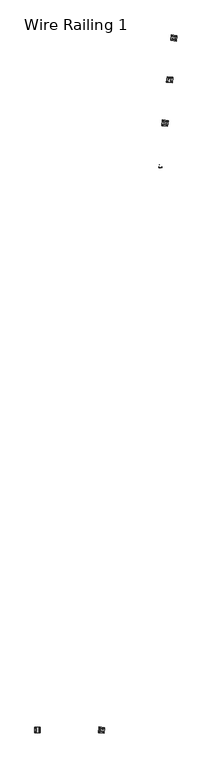
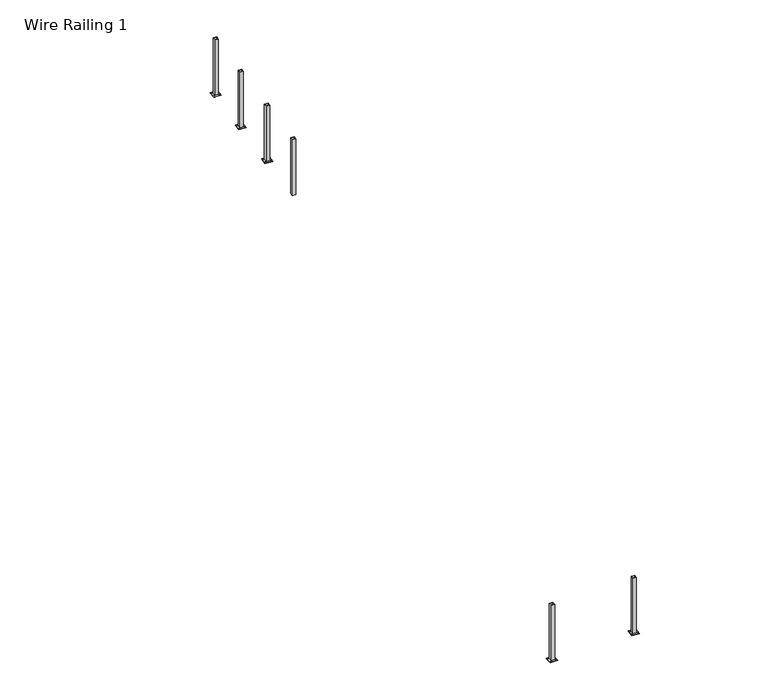
"""IFC4 building model written with IfcOpenShell, lengths in millimetres: railing geometry, Wire Railing 1."""

import ifcopenshell
import ifcopenshell.guid

model = None  # the IFC model being written
_history = None  # IfcOwnerHistory: only IFC2X3 demands one
_inside = {}  # id of a spatial element -> (the spatial element, [elements in it])
_under = {}  # id of a project, library or spatial element -> (it, [spatial elements below it])
_declared = {}  # id of a project -> (the project, [libraries it declares])
_typed = {}  # id of a type object -> (the type object, [elements of that type])
_made_of = {}  # id of a material, layer set ... -> (it, [elements and type objects made of it])


def new_model(schema):
    """Start an empty IFC model of exactly this schema.

    Asked for "IFC4X3", IfcOpenShell would pick the latest addendum, in which some entities
    have other attributes; the version numbers below select the first issue.
    IFC2X3 requires an IfcOwnerHistory on every rooted entity: one is made here for all.
    """
    global model, _history
    if schema == "IFC4X3":
        model = ifcopenshell.file(schema_version=(4, 3, 0, 0))
    else:
        model = ifcopenshell.file(schema=schema)
    _inside.clear()
    _under.clear()
    _declared.clear()
    _typed.clear()
    _made_of.clear()
    _history = None
    if model.schema == "IFC2X3":
        org = make("IfcOrganization", Name="unknown")
        user = make(
            "IfcPersonAndOrganization",
            ThePerson=make("IfcPerson", FamilyName="unknown"),
            TheOrganization=org,
        )
        app = make(
            "IfcApplication",
            ApplicationDeveloper=org,
            Version="unknown",
            ApplicationFullName="unknown",
            ApplicationIdentifier="unknown",
        )
        _history = make(
            "IfcOwnerHistory",
            OwningUser=user,
            OwningApplication=app,
            ChangeAction="ADDED",
            CreationDate=0,
        )
    return model


def make(cls, **values):
    """One entity of the class cls with the attributes given. An attribute that is None is left unset."""
    return model.create_entity(
        cls, **{name: value for name, value in values.items() if value is not None}
    )


def rooted(cls, **values):
    """An entity with a GlobalId (a new one), such as an element, a storey or a relation."""
    return make(cls, GlobalId=ifcopenshell.guid.new(), OwnerHistory=_history, **values)


def si_unit(unit_type, name, prefix=None):
    """IfcSIUnit, for example si_unit("LENGTHUNIT", "METRE", prefix="MILLI")."""
    return make("IfcSIUnit", UnitType=unit_type, Prefix=prefix, Name=name)


def assignment(units):
    """IfcUnitAssignment: the units of a project."""
    return None if units is None else make("IfcUnitAssignment", Units=units)


def point(xyz):
    """IfcCartesianPoint."""
    return None if xyz is None else make("IfcCartesianPoint", Coordinates=xyz)


def direction(xyz):
    """IfcDirection."""
    return None if xyz is None else make("IfcDirection", DirectionRatios=xyz)


def frame(location, z_axis=None, x_axis=None):
    """IfcAxis2Placement3D, a coordinate frame: its origin and axes. An axis left out is left unset."""
    return make(
        "IfcAxis2Placement3D",
        Location=point(location),
        Axis=direction(z_axis),
        RefDirection=direction(x_axis),
    )


def frame_2d(location, x_axis=None):
    """IfcAxis2Placement2D, a coordinate frame in the plane: its origin and x axis."""
    return make(
        "IfcAxis2Placement2D", Location=point(location), RefDirection=direction(x_axis)
    )


def origin():
    """The frame at (0, 0, 0) with its axes left unset."""
    return frame((0.0, 0.0, 0.0))


def place(relative_to, where):
    """IfcLocalPlacement: puts the frame where relative to a parent placement (None: the world)."""
    return make(
        "IfcLocalPlacement", PlacementRelTo=relative_to, RelativePlacement=where
    )


def context(
    kind, dimensions, precision=None, world=None, true_north=None, identifier=None
):
    """IfcGeometricRepresentationContext, for example the 3D "Model" context."""
    return make(
        "IfcGeometricRepresentationContext",
        ContextIdentifier=identifier,
        ContextType=kind,
        CoordinateSpaceDimension=dimensions,
        Precision=precision,
        WorldCoordinateSystem=world,
        TrueNorth=true_north,
    )


def project(units=None, contexts=None):
    """IfcProject with its units and contexts."""
    return rooted(
        "IfcProject",
        Name="project",
        RepresentationContexts=contexts,
        UnitsInContext=assignment(units),
    )


def spatial(cls, under=None, at=None, **own):
    """A site, building, storey or space (cls), placed at a placement, below another one or the project."""
    s = rooted(cls, ObjectPlacement=at, **own)
    if under is not None:
        _under.setdefault(under.id(), (under, []))[1].append(s)
    return s


def polyline(points):
    """IfcPolyline through the points."""
    return make("IfcPolyline", Points=[point(p) for p in points])


def circle_curve(where, radius):
    """IfcCircle in the frame where."""
    return make("IfcCircle", Position=where, Radius=radius)


def trimmed(basis, trim1, trim2, sense, master):
    """IfcTrimmedCurve: the piece of a basis curve between two trims."""
    return make(
        "IfcTrimmedCurve",
        BasisCurve=basis,
        Trim1=trim1,
        Trim2=trim2,
        SenseAgreement=sense,
        MasterRepresentation=master,
    )


def segment(curve, same_sense, transition):
    """IfcCompositeCurveSegment."""
    return make(
        "IfcCompositeCurveSegment",
        Transition=transition,
        SameSense=same_sense,
        ParentCurve=curve,
    )


def composite_curve(segments, self_intersect=None):
    """IfcCompositeCurve: segments joined end to end."""
    return make("IfcCompositeCurve", Segments=segments, SelfIntersect=self_intersect)


def outline(outer, holes=None, kind="AREA"):
    """IfcArbitraryClosedProfileDef: a profile drawn as a closed curve; with holes, ...WithVoids."""
    if holes is None:
        return make("IfcArbitraryClosedProfileDef", ProfileType=kind, OuterCurve=outer)
    return make(
        "IfcArbitraryProfileDefWithVoids",
        ProfileType=kind,
        OuterCurve=outer,
        InnerCurves=holes,
    )


def extrude(swept, where, along, depth):
    """IfcExtrudedAreaSolid: the profile swept, set in the frame where, extruded along a direction by depth."""
    return make(
        "IfcExtrudedAreaSolid",
        SweptArea=swept,
        Position=where,
        ExtrudedDirection=direction(along),
        Depth=depth,
    )


def shape(context_of_items, identifier, shape_type, items):
    """IfcShapeRepresentation: the items that make up one representation, for example the "Body"."""
    return make(
        "IfcShapeRepresentation",
        ContextOfItems=context_of_items,
        RepresentationIdentifier=identifier,
        RepresentationType=shape_type,
        Items=items,
    )


def source(mapping_origin, context_of_items, identifier, shape_type, items):
    """IfcRepresentationMap: a shape defined once, which mapped items show again and again."""
    return make(
        "IfcRepresentationMap",
        MappingOrigin=mapping_origin,
        MappedRepresentation=shape(context_of_items, identifier, shape_type, items),
    )


def transform(
    local_origin,
    x_axis=None,
    y_axis=None,
    z_axis=None,
    scale=None,
    scale2=None,
    scale3=None,
    uniform=True,
):
    """IfcCartesianTransformationOperator3D, or its non-uniform kind. x_axis, y_axis, z_axis: its Axis1, 2, 3."""
    if uniform:
        return make(
            "IfcCartesianTransformationOperator3D",
            Axis1=direction(x_axis),
            Axis2=direction(y_axis),
            LocalOrigin=point(local_origin),
            Scale=scale,
            Axis3=direction(z_axis),
        )
    return make(
        "IfcCartesianTransformationOperator3DnonUniform",
        Axis1=direction(x_axis),
        Axis2=direction(y_axis),
        LocalOrigin=point(local_origin),
        Scale=scale,
        Axis3=direction(z_axis),
        Scale2=scale2,
        Scale3=scale3,
    )


def mapped(mapping_source, mapping_target):
    """IfcMappedItem: shows the shape of a source again, moved by a transform."""
    return make(
        "IfcMappedItem", MappingSource=mapping_source, MappingTarget=mapping_target
    )


def made_of(thing, what):
    """Note that an element or type object is made of a material, layer set ...; save() writes the relation."""
    if what is not None:
        _made_of.setdefault(what.id(), (what, []))[1].append(thing)
    return thing


def element(
    cls,
    number,
    at=None,
    inside=None,
    cuts=None,
    type_object=None,
    material=None,
    context=None,
    identifier="Body",
    shape_type=None,
    held_by="IfcProductDefinitionShape",
    body=None,
    shapes=None,
    **own,
):
    """One element of the class cls, such as IfcWall. Its Tag is "e" and its number.

    at: its placement. inside: the storey or other place that contains it. cuts: it is an
    opening in that element (IfcRelVoidsElement). A single representation is given by context,
    identifier, shape_type and body (its items); several are given by shapes. held_by: the class
    of the entity that holds the representations. save() writes the other relations.
    """
    e = rooted(cls, Tag="e%d" % number, ObjectPlacement=at, **own)
    if body is not None:
        shapes = [shape(context, identifier, shape_type, body)]
    if shapes is not None:
        e.Representation = make(held_by, Representations=shapes)
    if inside is not None:
        _inside.setdefault(inside.id(), (inside, []))[1].append(e)
    if cuts is not None:
        rooted(
            "IfcRelVoidsElement", RelatingBuildingElement=cuts, RelatedOpeningElement=e
        )
    if type_object is not None:
        _typed.setdefault(type_object.id(), (type_object, []))[1].append(e)
    return made_of(e, material)


def aggregate(whole, parts):
    """IfcRelAggregates: a whole, such as a stair, and the parts it consists of."""
    return rooted("IfcRelAggregates", RelatingObject=whole, RelatedObjects=parts)


def save(model, path):
    """Write the relations noted so far, then the file.

    IfcRelAggregates (storeys below a building ...), IfcRelContainedInSpatialStructure (elements
    in a storey), IfcRelDefinesByType, IfcRelAssociatesMaterial and IfcRelDeclares: one each for
    every whole, place, type object, material and project.
    """
    for whole, parts in _under.values():
        aggregate(whole, parts)
    for where, things in _inside.values():
        rooted(
            "IfcRelContainedInSpatialStructure",
            RelatedElements=things,
            RelatingStructure=where,
        )
    for kind, things in _typed.values():
        rooted("IfcRelDefinesByType", RelatedObjects=things, RelatingType=kind)
    for what, things in _made_of.values():
        rooted("IfcRelAssociatesMaterial", RelatedObjects=things, RelatingMaterial=what)
    for by, libraries in _declared.values():
        rooted("IfcRelDeclares", RelatingContext=by, RelatedDefinitions=libraries)
    model.write(path)


def wire_railing_1_c7c1a042(model_context):
    return source(origin(), model_context, "Body", "SweptSolid", [
        extrude(outline(polyline([(35046.8311675, 38430.8279758), (35106.8257008, 38424.5222962), (35100.5200213, 38364.5277629), (35040.5254879, 38370.8334424), (35046.8311675, 38430.8279758)]), holes=[polyline([(35052.4826258, 38423.849006), (35047.5044577, 38376.4849007), (35094.868563, 38371.5067327), (35099.846731, 38418.8708379), (35052.4826258, 38423.849006)])]), frame((0.0, 0.0, 266395.2), z_axis=(0.0, 0.0, 1.0), x_axis=(1.0, 0.0, 0.0)), (0.0, 0.0, 1.0), 1047.75),
        extrude(outline(composite_curve([segment(trimmed(circle_curve(frame_2d((35226.1197211, 39422.8438242)), 6.35), [point((35232.4349351, 39422.1800684))], [point((35219.8045071, 39423.5075799))], False, "CARTESIAN"), True, "CONTINUOUS"), segment(trimmed(circle_curve(frame_2d((35226.1197211, 39422.8438242)), 6.35), [point((35219.8045071, 39423.5075799))], [point((35232.4349351, 39422.1800684))], False, "CARTESIAN"), True, "CONTINUOUS")], self_intersect=False)), frame((0.0, 0.0, 266395.2), z_axis=(0.0, 0.0, 1.0), x_axis=(1.0, 0.0, 0.0)), (0.0, 0.0, 1.0), 12.7),
        extrude(outline(composite_curve([segment(trimmed(circle_curve(frame_2d((35137.7067246, 39432.1364046)), 6.35), [point((35144.0219386, 39431.4726488))], [point((35131.3915106, 39432.8001603))], False, "CARTESIAN"), True, "CONTINUOUS"), segment(trimmed(circle_curve(frame_2d((35137.7067246, 39432.1364046)), 6.35), [point((35131.3915106, 39432.8001603))], [point((35144.0219386, 39431.4726488))], False, "CARTESIAN"), True, "CONTINUOUS")], self_intersect=False)), frame((0.0, 0.0, 266395.2), z_axis=(0.0, 0.0, 1.0), x_axis=(1.0, 0.0, 0.0)), (0.0, 0.0, 1.0), 12.7),
        extrude(outline(composite_curve([segment(trimmed(circle_curve(frame_2d((35216.8271407, 39334.4308277)), 6.35), [point((35223.1423547, 39333.7670719))], [point((35210.5119267, 39335.0945834))], False, "CARTESIAN"), True, "CONTINUOUS"), segment(trimmed(circle_curve(frame_2d((35216.8271407, 39334.4308277)), 6.35), [point((35210.5119267, 39335.0945834))], [point((35223.1423547, 39333.7670719))], False, "CARTESIAN"), True, "CONTINUOUS")], self_intersect=False)), frame((0.0, 0.0, 266395.2), z_axis=(0.0, 0.0, 1.0), x_axis=(1.0, 0.0, 0.0)), (0.0, 0.0, 1.0), 12.7),
        extrude(outline(composite_curve([segment(trimmed(circle_curve(frame_2d((35128.4141442, 39343.7234081)), 6.35), [point((35134.7293582, 39343.0596523))], [point((35122.0989302, 39344.3871638))], False, "CARTESIAN"), True, "CONTINUOUS"), segment(trimmed(circle_curve(frame_2d((35128.4141442, 39343.7234081)), 6.35), [point((35122.0989302, 39344.3871638))], [point((35134.7293582, 39343.0596523))], False, "CARTESIAN"), True, "CONTINUOUS")], self_intersect=False)), frame((0.0, 0.0, 266395.2), z_axis=(0.0, 0.0, 1.0), x_axis=(1.0, 0.0, 0.0)), (0.0, 0.0, 1.0), 12.7),
        extrude(outline(polyline([(35120.7523497, 39453.0733139), (35247.0566304, 39439.7981991), (35233.7815156, 39313.4939183), (35107.4772349, 39326.7690332), (35120.7523497, 39453.0733139)])), frame((0.0, 0.0, 266395.2), z_axis=(0.0, 0.0, 1.0), x_axis=(1.0, 0.0, 0.0)), (0.0, 0.0, 1.0), 6.35),
        extrude(outline(polyline([(35150.4225058, 39416.4337226), (35210.4170391, 39410.128043), (35204.1113595, 39350.1335097), (35144.1168262, 39356.4391892), (35150.4225058, 39416.4337226)]), holes=[polyline([(35156.073964, 39409.4547528), (35151.095796, 39362.0906475), (35198.4599013, 39357.1124794), (35203.4380693, 39404.4765847), (35156.073964, 39409.4547528)])]), frame((0.0, 0.0, 266395.2), z_axis=(0.0, 0.0, 1.0), x_axis=(1.0, 0.0, 0.0)), (0.0, 0.0, 1.0), 1047.75),
        extrude(outline(composite_curve([segment(trimmed(circle_curve(frame_2d((35329.7110594, 40408.4495709)), 6.35), [point((35336.0262734, 40407.7858152))], [point((35323.3958453, 40409.1133267))], False, "CARTESIAN"), True, "CONTINUOUS"), segment(trimmed(circle_curve(frame_2d((35329.7110594, 40408.4495709)), 6.35), [point((35323.3958453, 40409.1133267))], [point((35336.0262734, 40407.7858152))], False, "CARTESIAN"), True, "CONTINUOUS")], self_intersect=False)), frame((0.0, 0.0, 266395.2), z_axis=(0.0, 0.0, 1.0), x_axis=(1.0, 0.0, 0.0)), (0.0, 0.0, 1.0), 12.7),
        extrude(outline(composite_curve([segment(trimmed(circle_curve(frame_2d((35241.2980629, 40417.7421513)), 6.35), [point((35247.6132769, 40417.0783956))], [point((35234.9828488, 40418.4059071))], False, "CARTESIAN"), True, "CONTINUOUS"), segment(trimmed(circle_curve(frame_2d((35241.2980629, 40417.7421513)), 6.35), [point((35234.9828488, 40418.4059071))], [point((35247.6132769, 40417.0783956))], False, "CARTESIAN"), True, "CONTINUOUS")], self_intersect=False)), frame((0.0, 0.0, 266395.2), z_axis=(0.0, 0.0, 1.0), x_axis=(1.0, 0.0, 0.0)), (0.0, 0.0, 1.0), 12.7),
        extrude(outline(composite_curve([segment(trimmed(circle_curve(frame_2d((35320.418479, 40320.0365745)), 6.35), [point((35326.733693, 40319.3728187))], [point((35314.103265, 40320.7003302))], False, "CARTESIAN"), True, "CONTINUOUS"), segment(trimmed(circle_curve(frame_2d((35320.418479, 40320.0365745)), 6.35), [point((35314.103265, 40320.7003302))], [point((35326.733693, 40319.3728187))], False, "CARTESIAN"), True, "CONTINUOUS")], self_intersect=False)), frame((0.0, 0.0, 266395.2), z_axis=(0.0, 0.0, 1.0), x_axis=(1.0, 0.0, 0.0)), (0.0, 0.0, 1.0), 12.7),
        extrude(outline(composite_curve([segment(trimmed(circle_curve(frame_2d((35232.0054825, 40329.3291548)), 6.35), [point((35238.3206965, 40328.6653991))], [point((35225.6902685, 40329.9929106))], False, "CARTESIAN"), True, "CONTINUOUS"), segment(trimmed(circle_curve(frame_2d((35232.0054825, 40329.3291548)), 6.35), [point((35225.6902685, 40329.9929106))], [point((35238.3206965, 40328.6653991))], False, "CARTESIAN"), True, "CONTINUOUS")], self_intersect=False)), frame((0.0, 0.0, 266395.2), z_axis=(0.0, 0.0, 1.0), x_axis=(1.0, 0.0, 0.0)), (0.0, 0.0, 1.0), 12.7),
        extrude(outline(polyline([(35224.343688, 40438.6790607), (35350.6479687, 40425.4039458), (35337.3728539, 40299.0996651), (35211.0685732, 40312.37478), (35224.343688, 40438.6790607)])), frame((0.0, 0.0, 266395.2), z_axis=(0.0, 0.0, 1.0), x_axis=(1.0, 0.0, 0.0)), (0.0, 0.0, 1.0), 6.35),
        extrude(outline(polyline([(35254.013844, 40402.0394693), (35314.0083774, 40395.7337898), (35307.7026978, 40335.7392564), (35247.7081645, 40342.044936), (35254.013844, 40402.0394693)]), holes=[polyline([(35259.6653023, 40395.0604996), (35254.6871343, 40347.6963943), (35302.0512395, 40342.7182262), (35307.0294076, 40390.0823315), (35259.6653023, 40395.0604996)])]), frame((0.0, 0.0, 266395.2), z_axis=(0.0, 0.0, 1.0), x_axis=(1.0, 0.0, 0.0)), (0.0, 0.0, 1.0), 1047.75),
        extrude(outline(composite_curve([segment(trimmed(circle_curve(frame_2d((33775.840985, 25624.3633693)), 6.35), [point((33782.1561991, 25623.6996135))], [point((33769.525771, 25625.027125))], False, "CARTESIAN"), True, "CONTINUOUS"), segment(trimmed(circle_curve(frame_2d((33775.840985, 25624.3633693)), 6.35), [point((33769.525771, 25625.027125))], [point((33782.1561991, 25623.6996135))], False, "CARTESIAN"), True, "CONTINUOUS")], self_intersect=False)), frame((0.0, 0.0, 266395.2), z_axis=(0.0, 0.0, 1.0), x_axis=(1.0, 0.0, 0.0)), (0.0, 0.0, 1.0), 12.7),
        extrude(outline(composite_curve([segment(trimmed(circle_curve(frame_2d((33687.4279886, 25633.6559496)), 6.35), [point((33693.7432026, 25632.9921939))], [point((33681.1127745, 25634.3197054))], False, "CARTESIAN"), True, "CONTINUOUS"), segment(trimmed(circle_curve(frame_2d((33687.4279886, 25633.6559496)), 6.35), [point((33681.1127745, 25634.3197054))], [point((33693.7432026, 25632.9921939))], False, "CARTESIAN"), True, "CONTINUOUS")], self_intersect=False)), frame((0.0, 0.0, 266395.2), z_axis=(0.0, 0.0, 1.0), x_axis=(1.0, 0.0, 0.0)), (0.0, 0.0, 1.0), 12.7),
        extrude(outline(composite_curve([segment(trimmed(circle_curve(frame_2d((33766.5484047, 25535.9503728)), 6.35), [point((33772.8636187, 25535.286617))], [point((33760.2331906, 25536.6141285))], False, "CARTESIAN"), True, "CONTINUOUS"), segment(trimmed(circle_curve(frame_2d((33766.5484047, 25535.9503728)), 6.35), [point((33760.2331906, 25536.6141285))], [point((33772.8636187, 25535.286617))], False, "CARTESIAN"), True, "CONTINUOUS")], self_intersect=False)), frame((0.0, 0.0, 266395.2), z_axis=(0.0, 0.0, 1.0), x_axis=(1.0, 0.0, 0.0)), (0.0, 0.0, 1.0), 12.7),
        extrude(outline(composite_curve([segment(trimmed(circle_curve(frame_2d((33678.1354082, 25545.2429531)), 6.35), [point((33684.4506222, 25544.5791974))], [point((33671.8201941, 25545.9067089))], False, "CARTESIAN"), True, "CONTINUOUS"), segment(trimmed(circle_curve(frame_2d((33678.1354082, 25545.2429531)), 6.35), [point((33671.8201941, 25545.9067089))], [point((33684.4506222, 25544.5791974))], False, "CARTESIAN"), True, "CONTINUOUS")], self_intersect=False)), frame((0.0, 0.0, 266395.2), z_axis=(0.0, 0.0, 1.0), x_axis=(1.0, 0.0, 0.0)), (0.0, 0.0, 1.0), 12.7),
        extrude(outline(polyline([(33670.4736137, 25654.592859), (33796.7778944, 25641.3177441), (33783.5027795, 25515.0134634), (33657.1984988, 25528.2885783), (33670.4736137, 25654.592859)])), frame((0.0, 0.0, 266395.2), z_axis=(0.0, 0.0, 1.0), x_axis=(1.0, 0.0, 0.0)), (0.0, 0.0, 1.0), 6.35),
        extrude(outline(polyline([(33700.1437697, 25617.9532676), (33760.1383031, 25611.6475881), (33753.8326235, 25551.6530548), (33693.8380902, 25557.9587343), (33700.1437697, 25617.9532676)]), holes=[polyline([(33705.795228, 25610.9742979), (33700.8170599, 25563.6101926), (33748.1811652, 25558.6320245), (33753.1593333, 25605.9961298), (33705.795228, 25610.9742979)])]), frame((0.0, 0.0, 266395.2), z_axis=(0.0, 0.0, 1.0), x_axis=(1.0, 0.0, 0.0)), (0.0, 0.0, 1.0), 1047.75),
        extrude(outline(composite_curve([segment(trimmed(circle_curve(frame_2d((32317.2881966, 25540.3531612)), 6.35), [point((32317.2881966, 25534.0031612))], [point((32317.2881966, 25546.7031612))], False, "CARTESIAN"), True, "CONTINUOUS"), segment(trimmed(circle_curve(frame_2d((32317.2881966, 25540.3531612)), 6.35), [point((32317.2881966, 25546.7031612))], [point((32317.2881966, 25534.0031612))], False, "CARTESIAN"), True, "CONTINUOUS")], self_intersect=False)), frame((0.0, 0.0, 266395.2), z_axis=(0.0, 0.0, 1.0), x_axis=(1.0, 0.0, 0.0)), (0.0, 0.0, 1.0), 12.7),
        extrude(outline(composite_curve([segment(trimmed(circle_curve(frame_2d((32317.2881966, 25629.2531612)), 6.35), [point((32317.2881966, 25622.9031612))], [point((32317.2881966, 25635.6031612))], False, "CARTESIAN"), True, "CONTINUOUS"), segment(trimmed(circle_curve(frame_2d((32317.2881966, 25629.2531612)), 6.35), [point((32317.2881966, 25635.6031612))], [point((32317.2881966, 25622.9031612))], False, "CARTESIAN"), True, "CONTINUOUS")], self_intersect=False)), frame((0.0, 0.0, 266395.2), z_axis=(0.0, 0.0, 1.0), x_axis=(1.0, 0.0, 0.0)), (0.0, 0.0, 1.0), 12.7),
        extrude(outline(composite_curve([segment(trimmed(circle_curve(frame_2d((32228.3881966, 25540.3531612)), 6.35), [point((32228.3881966, 25534.0031612))], [point((32228.3881966, 25546.7031612))], False, "CARTESIAN"), True, "CONTINUOUS"), segment(trimmed(circle_curve(frame_2d((32228.3881966, 25540.3531612)), 6.35), [point((32228.3881966, 25546.7031612))], [point((32228.3881966, 25534.0031612))], False, "CARTESIAN"), True, "CONTINUOUS")], self_intersect=False)), frame((0.0, 0.0, 266395.2), z_axis=(0.0, 0.0, 1.0), x_axis=(1.0, 0.0, 0.0)), (0.0, 0.0, 1.0), 12.7),
        extrude(outline(composite_curve([segment(trimmed(circle_curve(frame_2d((32228.3881966, 25629.2531612)), 6.35), [point((32228.3881966, 25622.9031612))], [point((32228.3881966, 25635.6031612))], False, "CARTESIAN"), True, "CONTINUOUS"), segment(trimmed(circle_curve(frame_2d((32228.3881966, 25629.2531612)), 6.35), [point((32228.3881966, 25635.6031612))], [point((32228.3881966, 25622.9031612))], False, "CARTESIAN"), True, "CONTINUOUS")], self_intersect=False)), frame((0.0, 0.0, 266395.2), z_axis=(0.0, 0.0, 1.0), x_axis=(1.0, 0.0, 0.0)), (0.0, 0.0, 1.0), 12.7),
        extrude(outline(polyline([(32336.3381966, 25648.3031612), (32336.3381966, 25521.3031612), (32209.3381966, 25521.3031612), (32209.3381966, 25648.3031612), (32336.3381966, 25648.3031612)])), frame((0.0, 0.0, 266395.2), z_axis=(0.0, 0.0, 1.0), x_axis=(1.0, 0.0, 0.0)), (0.0, 0.0, 1.0), 6.35),
        extrude(outline(polyline([(32303.0006966, 25614.9656612), (32303.0006966, 25554.6406612), (32242.6756966, 25554.6406612), (32242.6756966, 25614.9656612), (32303.0006966, 25614.9656612)]), holes=[polyline([(32296.6506966, 25608.6156612), (32249.0256966, 25608.6156612), (32249.0256966, 25560.9906612), (32296.6506966, 25560.9906612), (32296.6506966, 25608.6156612)])]), frame((0.0, 0.0, 266395.2), z_axis=(0.0, 0.0, 1.0), x_axis=(1.0, 0.0, 0.0)), (0.0, 0.0, 1.0), 1047.75),
        extrude(outline(composite_curve([segment(trimmed(circle_curve(frame_2d((35429.3198632, 41356.1640335)), 6.35), [point((35435.6350773, 41355.5002778))], [point((35423.0046492, 41356.8277893))], False, "CARTESIAN"), True, "CONTINUOUS"), segment(trimmed(circle_curve(frame_2d((35429.3198632, 41356.1640335)), 6.35), [point((35423.0046492, 41356.8277893))], [point((35435.6350773, 41355.5002778))], False, "CARTESIAN"), True, "CONTINUOUS")], self_intersect=False)), frame((0.0, 0.0, 266395.2), z_axis=(0.0, 0.0, 1.0), x_axis=(1.0, 0.0, 0.0)), (0.0, 0.0, 1.0), 12.7),
        extrude(outline(composite_curve([segment(trimmed(circle_curve(frame_2d((35340.9068667, 41365.4566139)), 6.35), [point((35347.2220808, 41364.7928582))], [point((35334.5916527, 41366.1203696))], False, "CARTESIAN"), True, "CONTINUOUS"), segment(trimmed(circle_curve(frame_2d((35340.9068667, 41365.4566139)), 6.35), [point((35334.5916527, 41366.1203696))], [point((35347.2220808, 41364.7928582))], False, "CARTESIAN"), True, "CONTINUOUS")], self_intersect=False)), frame((0.0, 0.0, 266395.2), z_axis=(0.0, 0.0, 1.0), x_axis=(1.0, 0.0, 0.0)), (0.0, 0.0, 1.0), 12.7),
        extrude(outline(composite_curve([segment(trimmed(circle_curve(frame_2d((35420.0272828, 41267.751037)), 6.35), [point((35426.3424969, 41267.0872813))], [point((35413.7120688, 41268.4147928))], False, "CARTESIAN"), True, "CONTINUOUS"), segment(trimmed(circle_curve(frame_2d((35420.0272828, 41267.751037)), 6.35), [point((35413.7120688, 41268.4147928))], [point((35426.3424969, 41267.0872813))], False, "CARTESIAN"), True, "CONTINUOUS")], self_intersect=False)), frame((0.0, 0.0, 266395.2), z_axis=(0.0, 0.0, 1.0), x_axis=(1.0, 0.0, 0.0)), (0.0, 0.0, 1.0), 12.7),
        extrude(outline(composite_curve([segment(trimmed(circle_curve(frame_2d((35331.6142863, 41277.0436174)), 6.35), [point((35337.9295004, 41276.3798617))], [point((35325.2990723, 41277.7073731))], False, "CARTESIAN"), True, "CONTINUOUS"), segment(trimmed(circle_curve(frame_2d((35331.6142863, 41277.0436174)), 6.35), [point((35325.2990723, 41277.7073731))], [point((35337.9295004, 41276.3798617))], False, "CARTESIAN"), True, "CONTINUOUS")], self_intersect=False)), frame((0.0, 0.0, 266395.2), z_axis=(0.0, 0.0, 1.0), x_axis=(1.0, 0.0, 0.0)), (0.0, 0.0, 1.0), 12.7),
        extrude(outline(polyline([(35323.9524918, 41386.3935232), (35450.2567726, 41373.1184084), (35436.9816577, 41246.8141277), (35310.677377, 41260.0892425), (35323.9524918, 41386.3935232)])), frame((0.0, 0.0, 266395.2), z_axis=(0.0, 0.0, 1.0), x_axis=(1.0, 0.0, 0.0)), (0.0, 0.0, 1.0), 6.35),
        extrude(outline(polyline([(35353.6226479, 41349.7539319), (35413.6171812, 41343.4482524), (35407.3115017, 41283.453719), (35347.3169683, 41289.7593986), (35353.6226479, 41349.7539319)]), holes=[polyline([(35359.2741062, 41342.7749621), (35354.2959381, 41295.4108569), (35401.6600434, 41290.4326888), (35406.6382114, 41337.7967941), (35359.2741062, 41342.7749621)])]), frame((0.0, 0.0, 266395.2), z_axis=(0.0, 0.0, 1.0), x_axis=(1.0, 0.0, 0.0)), (0.0, 0.0, 1.0), 1047.75),
    ])


if __name__ == "__main__":
    model = new_model("IFC4")
    model_context = context("Model", 3, world=origin())
    ifc_project = project(units=[si_unit("LENGTHUNIT", "METRE", prefix="MILLI")], contexts=[model_context])
    site = spatial("IfcSite", under=ifc_project)
    building = spatial("IfcBuilding", under=site)
    placement = place(None, origin())
    wire_railing_1_shape = wire_railing_1_c7c1a042(model_context)
    element("IfcRailing", 1, ObjectType="Wire Railing 1", at=placement, inside=building, context=model_context, shape_type="MappedRepresentation", body=[
        mapped(wire_railing_1_shape, transform((0.0, 0.0, 0.0), x_axis=(1.0, 0.0, 0.0), y_axis=(0.0, 1.0, 0.0), z_axis=(0.0, 0.0, 1.0))),
    ])
    save(model, "model.ifc")

# Revit data of these elements
# Element 1 (IfcRailing, "Wire Railing 1")
#   Materials on its faces: "WIRE RAILING"
# Materials
#   "WIRE RAILING": class "Metal", colour RGB 244 244 244, transparency 0, Manufacturer = "Kawneer", URL = "http://www.kawneer.com/kawneer/north_america/en/home.asp", Cost = 0
